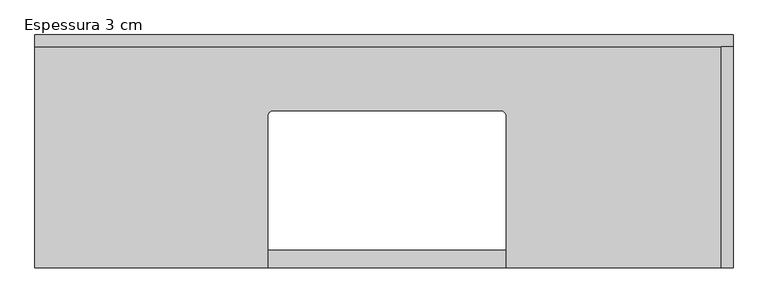
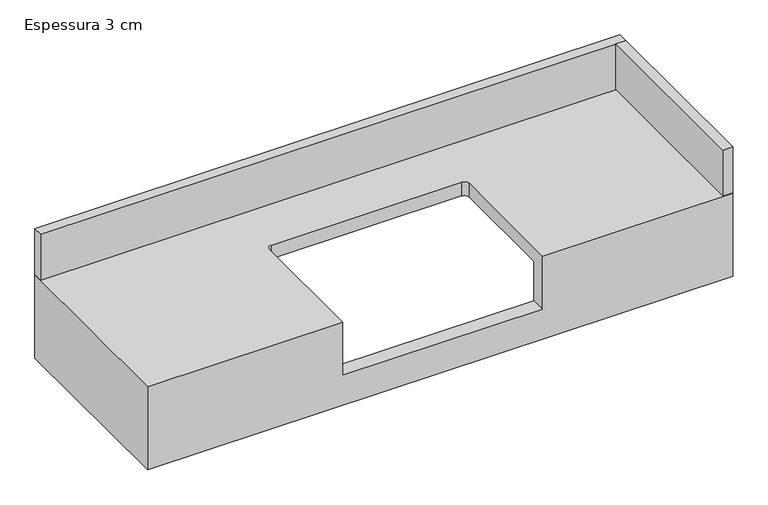
"""IFC4 building model written with IfcOpenShell, lengths in millimetres: furniture geometry, CC_BANCADA BANHEIRO COM CUBA_CANTO RETO : Espessura 3 cm."""

import ifcopenshell
import ifcopenshell.guid

model = None  # the IFC model being written
_history = None  # IfcOwnerHistory: only IFC2X3 demands one
_inside = {}  # id of a spatial element -> (the spatial element, [elements in it])
_under = {}  # id of a project, library or spatial element -> (it, [spatial elements below it])
_declared = {}  # id of a project -> (the project, [libraries it declares])
_typed = {}  # id of a type object -> (the type object, [elements of that type])
_made_of = {}  # id of a material, layer set ... -> (it, [elements and type objects made of it])


def new_model(schema):
    """Start an empty IFC model of exactly this schema.

    Asked for "IFC4X3", IfcOpenShell would pick the latest addendum, in which some entities
    have other attributes; the version numbers below select the first issue.
    IFC2X3 requires an IfcOwnerHistory on every rooted entity: one is made here for all.
    """
    global model, _history
    if schema == "IFC4X3":
        model = ifcopenshell.file(schema_version=(4, 3, 0, 0))
    else:
        model = ifcopenshell.file(schema=schema)
    _inside.clear()
    _under.clear()
    _declared.clear()
    _typed.clear()
    _made_of.clear()
    _history = None
    if model.schema == "IFC2X3":
        org = make("IfcOrganization", Name="unknown")
        user = make(
            "IfcPersonAndOrganization",
            ThePerson=make("IfcPerson", FamilyName="unknown"),
            TheOrganization=org,
        )
        app = make(
            "IfcApplication",
            ApplicationDeveloper=org,
            Version="unknown",
            ApplicationFullName="unknown",
            ApplicationIdentifier="unknown",
        )
        _history = make(
            "IfcOwnerHistory",
            OwningUser=user,
            OwningApplication=app,
            ChangeAction="ADDED",
            CreationDate=0,
        )
    return model


def make(cls, **values):
    """One entity of the class cls with the attributes given. An attribute that is None is left unset."""
    return model.create_entity(
        cls, **{name: value for name, value in values.items() if value is not None}
    )


def rooted(cls, **values):
    """An entity with a GlobalId (a new one), such as an element, a storey or a relation."""
    return make(cls, GlobalId=ifcopenshell.guid.new(), OwnerHistory=_history, **values)


def si_unit(unit_type, name, prefix=None):
    """IfcSIUnit, for example si_unit("LENGTHUNIT", "METRE", prefix="MILLI")."""
    return make("IfcSIUnit", UnitType=unit_type, Prefix=prefix, Name=name)


def assignment(units):
    """IfcUnitAssignment: the units of a project."""
    return None if units is None else make("IfcUnitAssignment", Units=units)


def point(xyz):
    """IfcCartesianPoint."""
    return None if xyz is None else make("IfcCartesianPoint", Coordinates=xyz)


def direction(xyz):
    """IfcDirection."""
    return None if xyz is None else make("IfcDirection", DirectionRatios=xyz)


def frame(location, z_axis=None, x_axis=None):
    """IfcAxis2Placement3D, a coordinate frame: its origin and axes. An axis left out is left unset."""
    return make(
        "IfcAxis2Placement3D",
        Location=point(location),
        Axis=direction(z_axis),
        RefDirection=direction(x_axis),
    )


def origin():
    """The frame at (0, 0, 0) with its axes left unset."""
    return frame((0.0, 0.0, 0.0))


def place(relative_to, where):
    """IfcLocalPlacement: puts the frame where relative to a parent placement (None: the world)."""
    return make(
        "IfcLocalPlacement", PlacementRelTo=relative_to, RelativePlacement=where
    )


def context(
    kind, dimensions, precision=None, world=None, true_north=None, identifier=None
):
    """IfcGeometricRepresentationContext, for example the 3D "Model" context."""
    return make(
        "IfcGeometricRepresentationContext",
        ContextIdentifier=identifier,
        ContextType=kind,
        CoordinateSpaceDimension=dimensions,
        Precision=precision,
        WorldCoordinateSystem=world,
        TrueNorth=true_north,
    )


def project(units=None, contexts=None):
    """IfcProject with its units and contexts."""
    return rooted(
        "IfcProject",
        Name="project",
        RepresentationContexts=contexts,
        UnitsInContext=assignment(units),
    )


def spatial(cls, under=None, at=None, **own):
    """A site, building, storey or space (cls), placed at a placement, below another one or the project."""
    s = rooted(cls, ObjectPlacement=at, **own)
    if under is not None:
        _under.setdefault(under.id(), (under, []))[1].append(s)
    return s


def polyline(points):
    """IfcPolyline through the points."""
    return make("IfcPolyline", Points=[point(p) for p in points])


def circle_curve(where, radius):
    """IfcCircle in the frame where."""
    return make("IfcCircle", Position=where, Radius=radius)


def outline(outer, holes=None, kind="AREA"):
    """IfcArbitraryClosedProfileDef: a profile drawn as a closed curve; with holes, ...WithVoids."""
    if holes is None:
        return make("IfcArbitraryClosedProfileDef", ProfileType=kind, OuterCurve=outer)
    return make(
        "IfcArbitraryProfileDefWithVoids",
        ProfileType=kind,
        OuterCurve=outer,
        InnerCurves=holes,
    )


def extrude(swept, where, along, depth):
    """IfcExtrudedAreaSolid: the profile swept, set in the frame where, extruded along a direction by depth."""
    return make(
        "IfcExtrudedAreaSolid",
        SweptArea=swept,
        Position=where,
        ExtrudedDirection=direction(along),
        Depth=depth,
    )


def shape(context_of_items, identifier, shape_type, items):
    """IfcShapeRepresentation: the items that make up one representation, for example the "Body"."""
    return make(
        "IfcShapeRepresentation",
        ContextOfItems=context_of_items,
        RepresentationIdentifier=identifier,
        RepresentationType=shape_type,
        Items=items,
    )


def source(mapping_origin, context_of_items, identifier, shape_type, items):
    """IfcRepresentationMap: a shape defined once, which mapped items show again and again."""
    return make(
        "IfcRepresentationMap",
        MappingOrigin=mapping_origin,
        MappedRepresentation=shape(context_of_items, identifier, shape_type, items),
    )


def transform(
    local_origin,
    x_axis=None,
    y_axis=None,
    z_axis=None,
    scale=None,
    scale2=None,
    scale3=None,
    uniform=True,
):
    """IfcCartesianTransformationOperator3D, or its non-uniform kind. x_axis, y_axis, z_axis: its Axis1, 2, 3."""
    if uniform:
        return make(
            "IfcCartesianTransformationOperator3D",
            Axis1=direction(x_axis),
            Axis2=direction(y_axis),
            LocalOrigin=point(local_origin),
            Scale=scale,
            Axis3=direction(z_axis),
        )
    return make(
        "IfcCartesianTransformationOperator3DnonUniform",
        Axis1=direction(x_axis),
        Axis2=direction(y_axis),
        LocalOrigin=point(local_origin),
        Scale=scale,
        Axis3=direction(z_axis),
        Scale2=scale2,
        Scale3=scale3,
    )


def mapped(mapping_source, mapping_target):
    """IfcMappedItem: shows the shape of a source again, moved by a transform."""
    return make(
        "IfcMappedItem", MappingSource=mapping_source, MappingTarget=mapping_target
    )


def made_of(thing, what):
    """Note that an element or type object is made of a material, layer set ...; save() writes the relation."""
    if what is not None:
        _made_of.setdefault(what.id(), (what, []))[1].append(thing)
    return thing


def element(
    cls,
    number,
    at=None,
    inside=None,
    cuts=None,
    type_object=None,
    material=None,
    context=None,
    identifier="Body",
    shape_type=None,
    held_by="IfcProductDefinitionShape",
    body=None,
    shapes=None,
    **own,
):
    """One element of the class cls, such as IfcWall. Its Tag is "e" and its number.

    at: its placement. inside: the storey or other place that contains it. cuts: it is an
    opening in that element (IfcRelVoidsElement). A single representation is given by context,
    identifier, shape_type and body (its items); several are given by shapes. held_by: the class
    of the entity that holds the representations. save() writes the other relations.
    """
    e = rooted(cls, Tag="e%d" % number, ObjectPlacement=at, **own)
    if body is not None:
        shapes = [shape(context, identifier, shape_type, body)]
    if shapes is not None:
        e.Representation = make(held_by, Representations=shapes)
    if inside is not None:
        _inside.setdefault(inside.id(), (inside, []))[1].append(e)
    if cuts is not None:
        rooted(
            "IfcRelVoidsElement", RelatingBuildingElement=cuts, RelatedOpeningElement=e
        )
    if type_object is not None:
        _typed.setdefault(type_object.id(), (type_object, []))[1].append(e)
    return made_of(e, material)


def aggregate(whole, parts):
    """IfcRelAggregates: a whole, such as a stair, and the parts it consists of."""
    return rooted("IfcRelAggregates", RelatingObject=whole, RelatedObjects=parts)


def save(model, path):
    """Write the relations noted so far, then the file.

    IfcRelAggregates (storeys below a building ...), IfcRelContainedInSpatialStructure (elements
    in a storey), IfcRelDefinesByType, IfcRelAssociatesMaterial and IfcRelDeclares: one each for
    every whole, place, type object, material and project.
    """
    for whole, parts in _under.values():
        aggregate(whole, parts)
    for where, things in _inside.values():
        rooted(
            "IfcRelContainedInSpatialStructure",
            RelatedElements=things,
            RelatingStructure=where,
        )
    for kind, things in _typed.values():
        rooted("IfcRelDefinesByType", RelatedObjects=things, RelatingType=kind)
    for what, things in _made_of.values():
        rooted("IfcRelAssociatesMaterial", RelatedObjects=things, RelatingMaterial=what)
    for by, libraries in _declared.values():
        rooted("IfcRelDeclares", RelatingContext=by, RelatedDefinitions=libraries)
    model.write(path)


def plane_surface(at):
    """IfcPlane: the flat surface through the origin of the frame at, square to its z axis."""
    return make("IfcPlane", Position=at)


def revolved_surface(curve, axis_point, axis_direction):
    """IfcSurfaceOfRevolution: the curve turned about the line through axis_point along axis_direction."""
    return make(
        "IfcSurfaceOfRevolution",
        SweptCurve=make("IfcArbitraryOpenProfileDef", ProfileType="CURVE", Curve=curve),
        AxisPosition=make("IfcAxis1Placement", Location=point(axis_point), Axis=direction(axis_direction)),
    )


def advanced_brep(points, edges, surfaces, faces):
    """IfcAdvancedBrep: a solid bounded by faces that lie on surfaces and meet in shared edges.

    An edge is (start, end): straight between two places in points (the first is 0);
    or (start, end, curve); or (start, end, curve, False) where it runs against its curve.
    A face is (place in surfaces, loops), or (place, loops, False) where it looks against
    its surface's normal. A loop lists edges by number (the first is 1), with a minus sign
    where the edge is run from its end to its start. The first loop is the outer one.
    """
    corners = [point(p) for p in points]
    vertices = [make("IfcVertexPoint", VertexGeometry=c) for c in corners]
    made = []
    for start, end, *more in edges:
        made.append(
            make(
                "IfcEdgeCurve",
                EdgeStart=vertices[start],
                EdgeEnd=vertices[end],
                EdgeGeometry=more[0] if more else make("IfcPolyline", Points=[corners[start], corners[end]]),
                SameSense=more[1] if len(more) > 1 else True,
            )
        )
    hull = []
    for where, loops, *sense in faces:
        bounds = []
        for j, loop in enumerate(loops):
            ring = [make("IfcOrientedEdge", EdgeElement=made[abs(k) - 1], Orientation=k > 0) for k in loop]
            bounds.append(
                make(
                    "IfcFaceOuterBound" if j == 0 else "IfcFaceBound",
                    Bound=make("IfcEdgeLoop", EdgeList=ring),
                    Orientation=True,
                )
            )
        hull.append(make("IfcAdvancedFace", Bounds=bounds, FaceSurface=surfaces[where], SameSense=sense[0] if sense else True))
    return make("IfcAdvancedBrep", Outer=make("IfcClosedShell", CfsFaces=hull))


def espessura_3_cm_493110b7(model_context):
    return source(origin(), model_context, "Body", "SolidModel", [
        advanced_brep(
        [(750.0, 300.0, 860.0), (-450.0, 300.0, 860.0), (-450.0, -100.0, 860.0), (-50.0, -100.0, 860.0), (-50.0, 160.0, 860.0), (-40.0, 170.0, 860.0), (350.0, 170.0, 860.0), (360.0, 160.0, 860.0), (360.0, -100.0, 860.0), (750.0, -100.0, 860.0), (750.0, 300.0, 680.0), (720.0, 300.0, 680.0), (720.0, 300.0, 830.0), (-420.0, 300.0, 830.0), (-420.0, 300.0, 680.0), (-450.0, 300.0, 680.0), (-450.0, -100.0, 680.0), (750.0, -100.0, 680.0), (360.0, -100.0, 745.0), (-50.0, -100.0, 745.0), (720.0, -70.0, 830.0), (360.0, -70.0, 830.0), (360.0, 160.0, 830.0), (350.0, 170.0, 830.0), (-40.0, 170.0, 830.0), (-50.0, 160.0, 830.0), (-50.0, -70.0, 830.0), (-420.0, -70.0, 830.0), (-420.0, -70.0, 680.0), (-50.0, -70.0, 745.0), (360.0, -70.0, 745.0), (720.0, -70.0, 680.0)],
        [
            (0, 1),
            (1, 2),
            (2, 3),
            (3, 4),
            (4, 5, circle_curve(frame((-40.0, 160.0, 860.0), z_axis=(0.0, 0.0, -1.0), x_axis=(0.0, 1.0, 0.0)), 10.0)),
            (5, 6),
            (6, 7, circle_curve(frame((350.0, 160.0, 860.0), z_axis=(0.0, 0.0, -1.0), x_axis=(0.0, 1.0, 0.0)), 10.0)),
            (7, 8),
            (8, 9),
            (9, 0),
            (0, 10),
            (10, 11),
            (11, 12),
            (12, 13),
            (13, 14),
            (14, 15),
            (15, 1),
            (15, 16),
            (16, 2),
            (16, 17),
            (17, 9),
            (8, 18),
            (18, 19),
            (19, 3),
            (17, 10),
            (12, 20),
            (20, 21),
            (21, 22),
            (22, 23, circle_curve(frame((350.0, 160.0, 830.0), z_axis=(0.0, 0.0, 1.0), x_axis=(0.0, 1.0, 0.0)), 10.0)),
            (23, 24),
            (24, 25, circle_curve(frame((-40.0, 160.0, 830.0), z_axis=(0.0, 0.0, 1.0), x_axis=(0.0, 1.0, 0.0)), 10.0)),
            (25, 26),
            (26, 27),
            (27, 13),
            (27, 28),
            (28, 14),
            (26, 29),
            (29, 30),
            (30, 21),
            (20, 31),
            (31, 28),
            (11, 31),
            (5, 24),
            (23, 6),
            (18, 30),
            (29, 19),
            (4, 25),
            (7, 22),
        ],
        [
            plane_surface(frame((-450.0, 300.0, 860.0), z_axis=(0.0, 0.0, 1.0), x_axis=(-1.0, 0.0, 0.0))),
            plane_surface(frame((750.0, 300.0, 860.0), z_axis=(0.0, 1.0, 0.0), x_axis=(0.0, 0.0, -1.0))),
            plane_surface(frame((-450.0, 300.0, 860.0), z_axis=(-1.0, 0.0, 0.0), x_axis=(0.0, 0.0, -1.0))),
            plane_surface(frame((-450.0, -100.0, 860.0), z_axis=(0.0, -1.0, 0.0), x_axis=(0.0, 0.0, -1.0))),
            plane_surface(frame((750.0, -100.0, 860.0), z_axis=(1.0, 0.0, 0.0), x_axis=(0.0, 0.0, -1.0))),
            plane_surface(frame((-420.0, 300.0, 830.0), z_axis=(0.0, 0.0, -1.0), x_axis=(-1.0, 0.0, 0.0))),
            plane_surface(frame((-420.0, 300.0, 830.0), z_axis=(1.0, 0.0, 0.0), x_axis=(0.0, 0.0, -1.0))),
            plane_surface(frame((-420.0, -70.0, 830.0), z_axis=(0.0, 1.0, 0.0), x_axis=(0.0, 0.0, -1.0))),
            plane_surface(frame((720.0, -70.0, 830.0), z_axis=(-1.0, 0.0, 0.0), x_axis=(0.0, 0.0, -1.0))),
            plane_surface(frame((750.0, -100.0, 680.0), z_axis=(0.0, 0.0, -1.0), x_axis=(0.0, 1.0, 0.0))),
            plane_surface(frame((-40.0, 170.0, 745.0), z_axis=(0.0, -1.0, 0.0), x_axis=(0.0, 0.0, 1.0))),
            plane_surface(frame((350.0, 170.0, 745.0), z_axis=(0.0, 0.0, 1.0), x_axis=(1.0, 0.0, 0.0))),
            revolved_surface(polyline([(-40.0, 170.0, 830.0), (-40.0, 170.0, 860.0)]), (-40.0, 160.0, 900.0), (0.0, 0.0, -1.0)),
            plane_surface(frame((-50.0, -230.0, 745.0), z_axis=(1.0, 0.0, 0.0), x_axis=(0.0, 0.0, 1.0))),
            plane_surface(frame((360.0, 160.0, 745.0), z_axis=(-1.0, 0.0, 0.0), x_axis=(0.0, 0.0, 1.0))),
            revolved_surface(polyline([(350.0, 170.0, 830.0), (350.0, 170.0, 860.0)]), (350.0, 160.0, 900.0), (0.0, 0.0, -1.0)),
        ],
        [
            (0, [[1, 2, 3, 4, 5, 6, 7, 8, 9, 10]]),
            (1, [[-1, 11, 12, 13, 14, 15, 16, 17]]),
            (2, [[-2, -17, 18, 19]]),
            (3, [[-3, -19, 20, 21, -9, 22, 23, 24]]),
            (4, [[-10, -21, 25, -11]]),
            (5, [[26, 27, 28, 29, 30, 31, 32, 33, 34, -14]]),
            (6, [[-34, 35, 36, -15]]),
            (7, [[-33, 37, 38, 39, -27, 40, 41, -35]]),
            (8, [[-26, -13, 42, -40]]),
            (9, [[-12, -25, -20, -18, -16, -36, -41, -42]]),
            (10, [[-6, 43, -30, 44]]),
            (11, [[-23, 45, -38, 46]]),
            (12, [[-5, 47, -31, -43]]),
            (13, [[-4, -24, -46, -37, -32, -47]]),
            (14, [[-8, 48, -28, -39, -45, -22]]),
            (15, [[-7, -44, -29, -48]]),
        ],
    ),
        extrude(outline(polyline([(730.0, 280.0), (750.0, 280.0), (750.0, -100.0), (730.0, -100.0), (730.0, 280.0)])), frame((0.0, 0.0, 860.0), z_axis=(0.0, 0.0, 1.0), x_axis=(1.0, 0.0, 0.0)), (0.0, 0.0, 1.0), 100.0),
        extrude(outline(polyline([(750.0, 300.0), (750.0, 280.0), (-450.0, 280.0), (-450.0, 300.0), (750.0, 300.0)])), frame((0.0, 0.0, 860.0), z_axis=(0.0, 0.0, 1.0), x_axis=(1.0, 0.0, 0.0)), (0.0, 0.0, 1.0), 100.0),
    ])


if __name__ == "__main__":
    model = new_model("IFC4")
    model_context = context("Model", 3, world=origin())
    ifc_project = project(units=[si_unit("LENGTHUNIT", "METRE", prefix="MILLI")], contexts=[model_context])
    site = spatial("IfcSite", under=ifc_project)
    building = spatial("IfcBuilding", under=site)
    placement = place(None, origin())
    espessura_3_cm_shape = espessura_3_cm_493110b7(model_context)
    element("IfcFurniture", 1, ObjectType="CC_BANCADA BANHEIRO COM CUBA_CANTO RETO : Espessura 3 cm", at=placement, inside=building, context=model_context, shape_type="MappedRepresentation", body=[
        mapped(espessura_3_cm_shape, transform((0.0, 0.0, 0.0), x_axis=(1.0, 0.0, 0.0), y_axis=(0.0, 1.0, 0.0), z_axis=(0.0, 0.0, 1.0))),
    ])
    save(model, "model.ifc")

# Revit data of these elements
# Type "CC_BANCADA BANHEIRO COM CUBA_CANTO RETO : Espessura 3 cm"
#   Uso HS [instance default] = ""
#   h TESTEIRA AUX [instance default] = 0.15 m
#   Altura testeira [instance default] = 0.15 m
#   Altura rodapia [instance default] = 0.10 m
#   Espessura rodapia [instance default] = 0.02 m
#   Prof/2 [instance default] = 0.20 m
#   Offset cuba esquerda [instance default] = 0.40 m
#   Depth [instance default] = 1.20 m
#   Width [instance default] = 0.40 m
#   Espessura bancada = 0.03 m
#   Comprimento [instance default] = 1.20 m
#   Height [instance default] = 0.86 m
#   Testeira [instance default] = yes
#   Rodapia fundo [instance default] = no
#   Rodapia esquerda [instance default] = no
#   Rodapia direita [instance default] = no
#   Material porta-toalha [instance default] = .CROMADO
#   Material hidráulico [instance default] = .CROMADO
#   Material cuba [instance default] = .PORCELANA BRANCA
#   Material bancada [instance default] = .GRANITO_BRANCO_ITAUNAS
#   Assembly Code = ""
# Element 1 (IfcFurniture, "CC_BANCADA BANHEIRO COM CUBA_CANTO RETO : Espessura 3 cm")
#   Uso HS = "BANHO SUÍTE 1"
#   Rodapia fundo = yes
#   Rodapia direita = yes
#   Materials on its faces: ".GRANITO_BRANCO_ITAUNAS"
# Materials
#   ".CROMADO": class "CC_METAIS", colour RGB 211 223 226, transparency 0, Cost = 0
#   ".PORCELANA BRANCA": class "CC_PORCELANA", colour RGB 230 230 230, transparency 0, Cost = 0
#   ".GRANITO_BRANCO_ITAUNAS": class ".CC_PEDRA REVEST.", colour RGB 202 195 174, transparency 0, Description = "Revestimento em granito", Cost = 0
